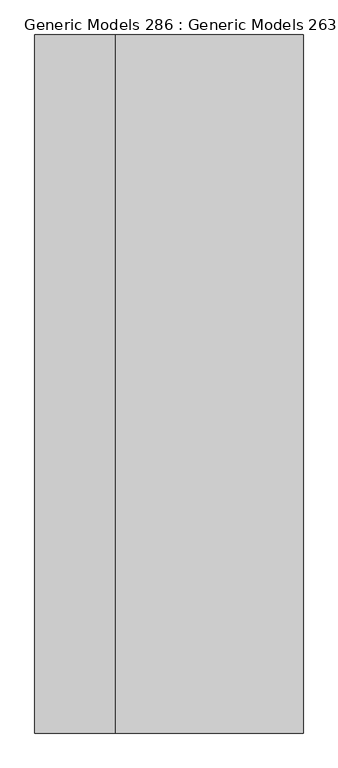
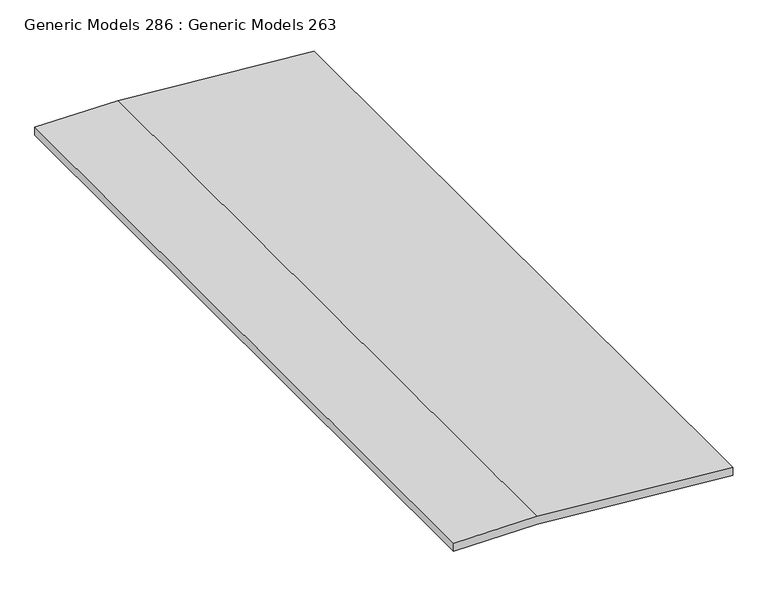
"""IFC4 building model written with IfcOpenShell, lengths in millimetres: proxy geometry, Generic Models 286 : Generic Models 263."""

from ifc_helpers import new_model, si_unit, frame, origin, place, context, project, spatial, polyline, outline, extrude, source, transform, mapped, element, save


def generic_models_286_generic_models_263_f82cf649(model_context):
    return source(origin(), model_context, "Body", "SweptSolid", [
        extrude(outline(polyline([(-18.0020399, 88031.3862389), (0.2818898, 86515.9481279), (-152.129202, 86515.9481279), (-170.3245887, 88024.0474769), (-470.5124436, 91579.9797726), (-317.5703646, 91579.9797726), (-18.0020399, 88031.3862389)])), frame((0.0, -6927.5236352, 0.0), z_axis=(0.0, 1.0, 0.0), x_axis=(0.0, 0.0, 1.0)), (0.0, 0.0, 1.0), 13159.4929723),
    ])


if __name__ == "__main__":
    model = new_model("IFC4")
    model_context = context("Model", 3, world=origin())
    ifc_project = project(units=[si_unit("LENGTHUNIT", "METRE", prefix="MILLI")], contexts=[model_context])
    site = spatial("IfcSite", under=ifc_project)
    building = spatial("IfcBuilding", under=site)
    placement = place(None, origin())
    generic_models_286_generic_models_263_shape = generic_models_286_generic_models_263_f82cf649(model_context)
    element("IfcBuildingElementProxy", 1, Name="Generic Models 286 : Generic Models 263", ObjectType="Generic Models 286 : Generic Models 263", at=placement, inside=building, context=model_context, shape_type="MappedRepresentation", body=[
        mapped(generic_models_286_generic_models_263_shape, transform((0.0, 0.0, 0.0), x_axis=(1.0, 0.0, 0.0), y_axis=(0.0, 1.0, 0.0), z_axis=(0.0, 0.0, 1.0))),
    ])
    save(model, "model.ifc")

# Revit data of these elements
# Element 1 (IfcBuildingElementProxy, "Generic Models 286 : Generic Models 263")
#   Materials on its faces: "6\" CRUSHED AGGREGATE BASE COURSE"
# Materials
#   "6\" CRUSHED AGGREGATE BASE COURSE": class "Miscellaneous", colour RGB 167 168 186, transparency 0, Cost = 0
